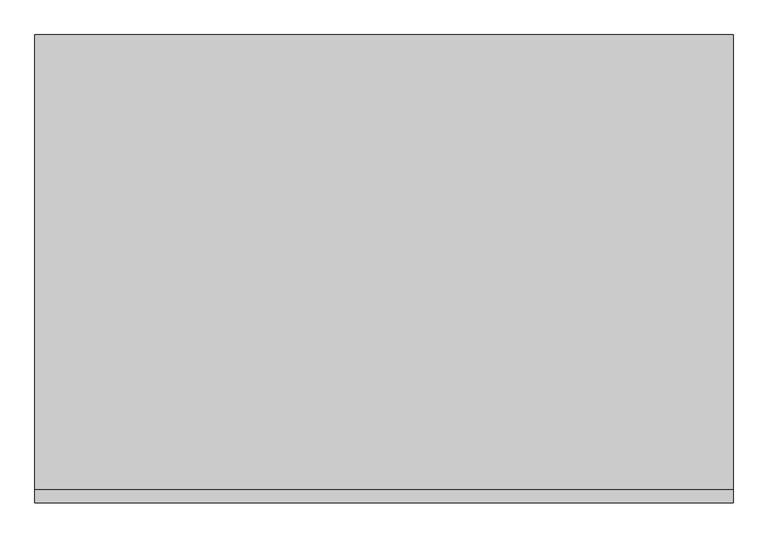
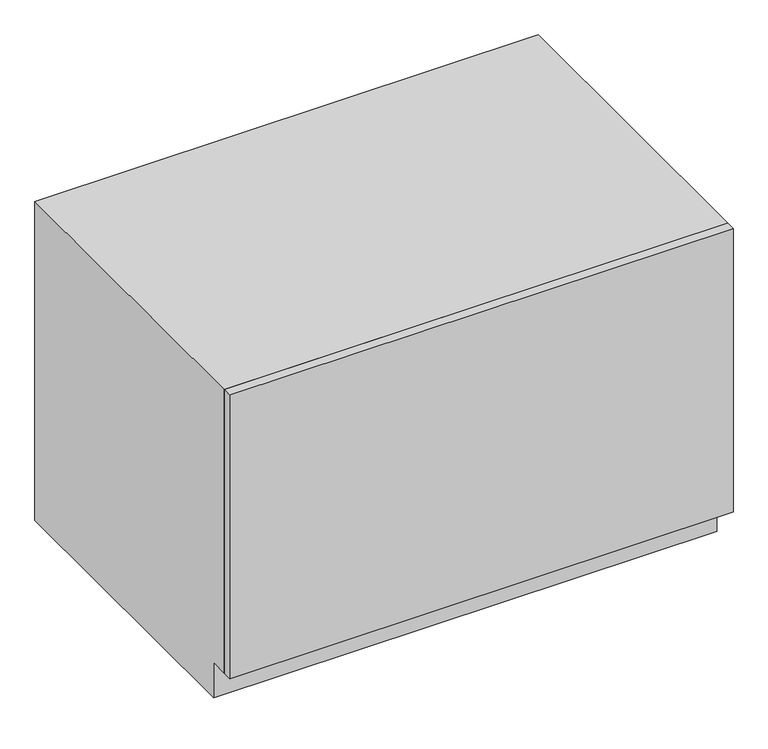
"""IFC4 building model written with IfcOpenShell, lengths in millimetres: furniture geometry, OD_CW_Base Cabinet : OD_CW_Base Cabinet."""

import ifcopenshell
import ifcopenshell.guid

model = None  # the IFC model being written
_history = None  # IfcOwnerHistory: only IFC2X3 demands one
_inside = {}  # id of a spatial element -> (the spatial element, [elements in it])
_under = {}  # id of a project, library or spatial element -> (it, [spatial elements below it])
_declared = {}  # id of a project -> (the project, [libraries it declares])
_typed = {}  # id of a type object -> (the type object, [elements of that type])
_made_of = {}  # id of a material, layer set ... -> (it, [elements and type objects made of it])


def new_model(schema):
    """Start an empty IFC model of exactly this schema.

    Asked for "IFC4X3", IfcOpenShell would pick the latest addendum, in which some entities
    have other attributes; the version numbers below select the first issue.
    IFC2X3 requires an IfcOwnerHistory on every rooted entity: one is made here for all.
    """
    global model, _history
    if schema == "IFC4X3":
        model = ifcopenshell.file(schema_version=(4, 3, 0, 0))
    else:
        model = ifcopenshell.file(schema=schema)
    _inside.clear()
    _under.clear()
    _declared.clear()
    _typed.clear()
    _made_of.clear()
    _history = None
    if model.schema == "IFC2X3":
        org = make("IfcOrganization", Name="unknown")
        user = make(
            "IfcPersonAndOrganization",
            ThePerson=make("IfcPerson", FamilyName="unknown"),
            TheOrganization=org,
        )
        app = make(
            "IfcApplication",
            ApplicationDeveloper=org,
            Version="unknown",
            ApplicationFullName="unknown",
            ApplicationIdentifier="unknown",
        )
        _history = make(
            "IfcOwnerHistory",
            OwningUser=user,
            OwningApplication=app,
            ChangeAction="ADDED",
            CreationDate=0,
        )
    return model


def make(cls, **values):
    """One entity of the class cls with the attributes given. An attribute that is None is left unset."""
    return model.create_entity(
        cls, **{name: value for name, value in values.items() if value is not None}
    )


def rooted(cls, **values):
    """An entity with a GlobalId (a new one), such as an element, a storey or a relation."""
    return make(cls, GlobalId=ifcopenshell.guid.new(), OwnerHistory=_history, **values)


def si_unit(unit_type, name, prefix=None):
    """IfcSIUnit, for example si_unit("LENGTHUNIT", "METRE", prefix="MILLI")."""
    return make("IfcSIUnit", UnitType=unit_type, Prefix=prefix, Name=name)


def assignment(units):
    """IfcUnitAssignment: the units of a project."""
    return None if units is None else make("IfcUnitAssignment", Units=units)


def point(xyz):
    """IfcCartesianPoint."""
    return None if xyz is None else make("IfcCartesianPoint", Coordinates=xyz)


def direction(xyz):
    """IfcDirection."""
    return None if xyz is None else make("IfcDirection", DirectionRatios=xyz)


def frame(location, z_axis=None, x_axis=None):
    """IfcAxis2Placement3D, a coordinate frame: its origin and axes. An axis left out is left unset."""
    return make(
        "IfcAxis2Placement3D",
        Location=point(location),
        Axis=direction(z_axis),
        RefDirection=direction(x_axis),
    )


def origin():
    """The frame at (0, 0, 0) with its axes left unset."""
    return frame((0.0, 0.0, 0.0))


def place(relative_to, where):
    """IfcLocalPlacement: puts the frame where relative to a parent placement (None: the world)."""
    return make(
        "IfcLocalPlacement", PlacementRelTo=relative_to, RelativePlacement=where
    )


def context(
    kind, dimensions, precision=None, world=None, true_north=None, identifier=None
):
    """IfcGeometricRepresentationContext, for example the 3D "Model" context."""
    return make(
        "IfcGeometricRepresentationContext",
        ContextIdentifier=identifier,
        ContextType=kind,
        CoordinateSpaceDimension=dimensions,
        Precision=precision,
        WorldCoordinateSystem=world,
        TrueNorth=true_north,
    )


def project(units=None, contexts=None):
    """IfcProject with its units and contexts."""
    return rooted(
        "IfcProject",
        Name="project",
        RepresentationContexts=contexts,
        UnitsInContext=assignment(units),
    )


def spatial(cls, under=None, at=None, **own):
    """A site, building, storey or space (cls), placed at a placement, below another one or the project."""
    s = rooted(cls, ObjectPlacement=at, **own)
    if under is not None:
        _under.setdefault(under.id(), (under, []))[1].append(s)
    return s


def polyline(points):
    """IfcPolyline through the points."""
    return make("IfcPolyline", Points=[point(p) for p in points])


def outline(outer, holes=None, kind="AREA"):
    """IfcArbitraryClosedProfileDef: a profile drawn as a closed curve; with holes, ...WithVoids."""
    if holes is None:
        return make("IfcArbitraryClosedProfileDef", ProfileType=kind, OuterCurve=outer)
    return make(
        "IfcArbitraryProfileDefWithVoids",
        ProfileType=kind,
        OuterCurve=outer,
        InnerCurves=holes,
    )


def extrude(swept, where, along, depth):
    """IfcExtrudedAreaSolid: the profile swept, set in the frame where, extruded along a direction by depth."""
    return make(
        "IfcExtrudedAreaSolid",
        SweptArea=swept,
        Position=where,
        ExtrudedDirection=direction(along),
        Depth=depth,
    )


def shape(context_of_items, identifier, shape_type, items):
    """IfcShapeRepresentation: the items that make up one representation, for example the "Body"."""
    return make(
        "IfcShapeRepresentation",
        ContextOfItems=context_of_items,
        RepresentationIdentifier=identifier,
        RepresentationType=shape_type,
        Items=items,
    )


def source(mapping_origin, context_of_items, identifier, shape_type, items):
    """IfcRepresentationMap: a shape defined once, which mapped items show again and again."""
    return make(
        "IfcRepresentationMap",
        MappingOrigin=mapping_origin,
        MappedRepresentation=shape(context_of_items, identifier, shape_type, items),
    )


def transform(
    local_origin,
    x_axis=None,
    y_axis=None,
    z_axis=None,
    scale=None,
    scale2=None,
    scale3=None,
    uniform=True,
):
    """IfcCartesianTransformationOperator3D, or its non-uniform kind. x_axis, y_axis, z_axis: its Axis1, 2, 3."""
    if uniform:
        return make(
            "IfcCartesianTransformationOperator3D",
            Axis1=direction(x_axis),
            Axis2=direction(y_axis),
            LocalOrigin=point(local_origin),
            Scale=scale,
            Axis3=direction(z_axis),
        )
    return make(
        "IfcCartesianTransformationOperator3DnonUniform",
        Axis1=direction(x_axis),
        Axis2=direction(y_axis),
        LocalOrigin=point(local_origin),
        Scale=scale,
        Axis3=direction(z_axis),
        Scale2=scale2,
        Scale3=scale3,
    )


def mapped(mapping_source, mapping_target):
    """IfcMappedItem: shows the shape of a source again, moved by a transform."""
    return make(
        "IfcMappedItem", MappingSource=mapping_source, MappingTarget=mapping_target
    )


def made_of(thing, what):
    """Note that an element or type object is made of a material, layer set ...; save() writes the relation."""
    if what is not None:
        _made_of.setdefault(what.id(), (what, []))[1].append(thing)
    return thing


def element(
    cls,
    number,
    at=None,
    inside=None,
    cuts=None,
    type_object=None,
    material=None,
    context=None,
    identifier="Body",
    shape_type=None,
    held_by="IfcProductDefinitionShape",
    body=None,
    shapes=None,
    **own,
):
    """One element of the class cls, such as IfcWall. Its Tag is "e" and its number.

    at: its placement. inside: the storey or other place that contains it. cuts: it is an
    opening in that element (IfcRelVoidsElement). A single representation is given by context,
    identifier, shape_type and body (its items); several are given by shapes. held_by: the class
    of the entity that holds the representations. save() writes the other relations.
    """
    e = rooted(cls, Tag="e%d" % number, ObjectPlacement=at, **own)
    if body is not None:
        shapes = [shape(context, identifier, shape_type, body)]
    if shapes is not None:
        e.Representation = make(held_by, Representations=shapes)
    if inside is not None:
        _inside.setdefault(inside.id(), (inside, []))[1].append(e)
    if cuts is not None:
        rooted(
            "IfcRelVoidsElement", RelatingBuildingElement=cuts, RelatedOpeningElement=e
        )
    if type_object is not None:
        _typed.setdefault(type_object.id(), (type_object, []))[1].append(e)
    return made_of(e, material)


def aggregate(whole, parts):
    """IfcRelAggregates: a whole, such as a stair, and the parts it consists of."""
    return rooted("IfcRelAggregates", RelatingObject=whole, RelatedObjects=parts)


def save(model, path):
    """Write the relations noted so far, then the file.

    IfcRelAggregates (storeys below a building ...), IfcRelContainedInSpatialStructure (elements
    in a storey), IfcRelDefinesByType, IfcRelAssociatesMaterial and IfcRelDeclares: one each for
    every whole, place, type object, material and project.
    """
    for whole, parts in _under.values():
        aggregate(whole, parts)
    for where, things in _inside.values():
        rooted(
            "IfcRelContainedInSpatialStructure",
            RelatedElements=things,
            RelatingStructure=where,
        )
    for kind, things in _typed.values():
        rooted("IfcRelDefinesByType", RelatedObjects=things, RelatingType=kind)
    for what, things in _made_of.values():
        rooted("IfcRelAssociatesMaterial", RelatedObjects=things, RelatingMaterial=what)
    for by, libraries in _declared.values():
        rooted("IfcRelDeclares", RelatingContext=by, RelatedDefinitions=libraries)
    model.write(path)


def furniture_e23802ca(model_context):
    return source(origin(), model_context, "Body", "SweptSolid", [
        extrude(outline(polyline([(18.7377049, -279.4), (1381.8947317, -279.4), (1381.8947317, -304.8), (18.7377049, -304.8), (18.7377049, -279.4)])), frame((0.0, 0.0, 101.6), z_axis=(0.0, 0.0, 1.0), x_axis=(1.0, 0.0, 0.0)), (0.0, 0.0, 1.0), 812.8),
        extrude(outline(polyline([(-279.4, 914.4), (609.6, 914.4), (609.6, 0.0), (-228.6, 0.0), (-228.6, 101.6), (-279.4, 101.6), (-279.4, 914.4)])), frame((18.7377049, 0.0, 0.0), z_axis=(1.0, 0.0, 0.0), x_axis=(0.0, 1.0, 0.0)), (0.0, 0.0, 1.0), 1363.1570268),
    ])


if __name__ == "__main__":
    model = new_model("IFC4")
    model_context = context("Model", 3, world=origin())
    ifc_project = project(units=[si_unit("LENGTHUNIT", "METRE", prefix="MILLI")], contexts=[model_context])
    site = spatial("IfcSite", under=ifc_project)
    building = spatial("IfcBuilding", under=site)
    placement = place(None, origin())
    furniture_shape = furniture_e23802ca(model_context)
    element("IfcFurniture", 1, ObjectType="OD_CW_Base Cabinet : OD_CW_Base Cabinet", at=placement, inside=building, context=model_context, shape_type="MappedRepresentation", body=[
        mapped(furniture_shape, transform((0.0, 0.0, 0.0), x_axis=(1.0, 0.0, 0.0), y_axis=(0.0, 1.0, 0.0), z_axis=(0.0, 0.0, 1.0))),
    ])
    save(model, "model.ifc")

# Revit data of these elements
# Type "OD_CW_Base Cabinet : OD_CW_Base Cabinet"
#   OD_CW_Width [instance default] = 2' - 10"
#   OD_CW_Length [instance default] = 8' - 0"
#   OD_CW_Height [instance default] = 2' - 3"
#   Depth = 2' - 0"
#   Height = 3' - 0"
#   Width = 4' - 0"
#   OD_CW_Material_Front Panel [instance default] = none
#   OD_CW_Material_Body [instance default] = none
# Element 1 (IfcFurniture, "OD_CW_Base Cabinet : OD_CW_Base Cabinet")
#   OD_CW_Width = 3' - 0"
#   OD_CW_Length = 4' - 5.6676"
#   OD_CW_Height = 3' - 0"
#   OD_CW_Material_Body = PANTRY RAIL
#   Materials on its faces: "PANTRY RAIL", "CASEWORK"
# Materials
#   "PANTRY RAIL": class "Generic", colour RGB 187 187 187, transparency 0, Cost = 0
#   "CASEWORK": class "Generic", colour RGB 181 181 181, transparency 0, Cost = 0
